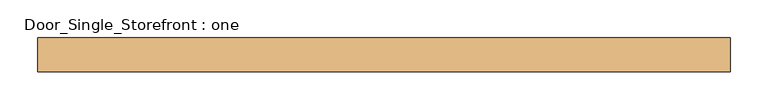
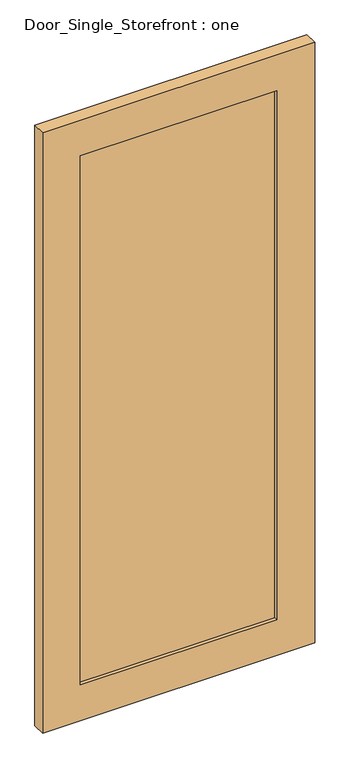
"""IFC4 building model written with IfcOpenShell, lengths in millimetres: door geometry, Door_Single_Storefront : one."""

import ifcopenshell
import ifcopenshell.guid

model = None  # the IFC model being written
_history = None  # IfcOwnerHistory: only IFC2X3 demands one
_inside = {}  # id of a spatial element -> (the spatial element, [elements in it])
_under = {}  # id of a project, library or spatial element -> (it, [spatial elements below it])
_declared = {}  # id of a project -> (the project, [libraries it declares])
_typed = {}  # id of a type object -> (the type object, [elements of that type])
_made_of = {}  # id of a material, layer set ... -> (it, [elements and type objects made of it])


def new_model(schema):
    """Start an empty IFC model of exactly this schema.

    Asked for "IFC4X3", IfcOpenShell would pick the latest addendum, in which some entities
    have other attributes; the version numbers below select the first issue.
    IFC2X3 requires an IfcOwnerHistory on every rooted entity: one is made here for all.
    """
    global model, _history
    if schema == "IFC4X3":
        model = ifcopenshell.file(schema_version=(4, 3, 0, 0))
    else:
        model = ifcopenshell.file(schema=schema)
    _inside.clear()
    _under.clear()
    _declared.clear()
    _typed.clear()
    _made_of.clear()
    _history = None
    if model.schema == "IFC2X3":
        org = make("IfcOrganization", Name="unknown")
        user = make(
            "IfcPersonAndOrganization",
            ThePerson=make("IfcPerson", FamilyName="unknown"),
            TheOrganization=org,
        )
        app = make(
            "IfcApplication",
            ApplicationDeveloper=org,
            Version="unknown",
            ApplicationFullName="unknown",
            ApplicationIdentifier="unknown",
        )
        _history = make(
            "IfcOwnerHistory",
            OwningUser=user,
            OwningApplication=app,
            ChangeAction="ADDED",
            CreationDate=0,
        )
    return model


def make(cls, **values):
    """One entity of the class cls with the attributes given. An attribute that is None is left unset."""
    return model.create_entity(
        cls, **{name: value for name, value in values.items() if value is not None}
    )


def rooted(cls, **values):
    """An entity with a GlobalId (a new one), such as an element, a storey or a relation."""
    return make(cls, GlobalId=ifcopenshell.guid.new(), OwnerHistory=_history, **values)


def si_unit(unit_type, name, prefix=None):
    """IfcSIUnit, for example si_unit("LENGTHUNIT", "METRE", prefix="MILLI")."""
    return make("IfcSIUnit", UnitType=unit_type, Prefix=prefix, Name=name)


def assignment(units):
    """IfcUnitAssignment: the units of a project."""
    return None if units is None else make("IfcUnitAssignment", Units=units)


def point(xyz):
    """IfcCartesianPoint."""
    return None if xyz is None else make("IfcCartesianPoint", Coordinates=xyz)


def direction(xyz):
    """IfcDirection."""
    return None if xyz is None else make("IfcDirection", DirectionRatios=xyz)


def frame(location, z_axis=None, x_axis=None):
    """IfcAxis2Placement3D, a coordinate frame: its origin and axes. An axis left out is left unset."""
    return make(
        "IfcAxis2Placement3D",
        Location=point(location),
        Axis=direction(z_axis),
        RefDirection=direction(x_axis),
    )


def origin():
    """The frame at (0, 0, 0) with its axes left unset."""
    return frame((0.0, 0.0, 0.0))


def place(relative_to, where):
    """IfcLocalPlacement: puts the frame where relative to a parent placement (None: the world)."""
    return make(
        "IfcLocalPlacement", PlacementRelTo=relative_to, RelativePlacement=where
    )


def context(
    kind, dimensions, precision=None, world=None, true_north=None, identifier=None
):
    """IfcGeometricRepresentationContext, for example the 3D "Model" context."""
    return make(
        "IfcGeometricRepresentationContext",
        ContextIdentifier=identifier,
        ContextType=kind,
        CoordinateSpaceDimension=dimensions,
        Precision=precision,
        WorldCoordinateSystem=world,
        TrueNorth=true_north,
    )


def project(units=None, contexts=None):
    """IfcProject with its units and contexts."""
    return rooted(
        "IfcProject",
        Name="project",
        RepresentationContexts=contexts,
        UnitsInContext=assignment(units),
    )


def spatial(cls, under=None, at=None, **own):
    """A site, building, storey or space (cls), placed at a placement, below another one or the project."""
    s = rooted(cls, ObjectPlacement=at, **own)
    if under is not None:
        _under.setdefault(under.id(), (under, []))[1].append(s)
    return s


def polyline(points):
    """IfcPolyline through the points."""
    return make("IfcPolyline", Points=[point(p) for p in points])


def outline(outer, holes=None, kind="AREA"):
    """IfcArbitraryClosedProfileDef: a profile drawn as a closed curve; with holes, ...WithVoids."""
    if holes is None:
        return make("IfcArbitraryClosedProfileDef", ProfileType=kind, OuterCurve=outer)
    return make(
        "IfcArbitraryProfileDefWithVoids",
        ProfileType=kind,
        OuterCurve=outer,
        InnerCurves=holes,
    )


def extrude(swept, where, along, depth):
    """IfcExtrudedAreaSolid: the profile swept, set in the frame where, extruded along a direction by depth."""
    return make(
        "IfcExtrudedAreaSolid",
        SweptArea=swept,
        Position=where,
        ExtrudedDirection=direction(along),
        Depth=depth,
    )


def shape(context_of_items, identifier, shape_type, items):
    """IfcShapeRepresentation: the items that make up one representation, for example the "Body"."""
    return make(
        "IfcShapeRepresentation",
        ContextOfItems=context_of_items,
        RepresentationIdentifier=identifier,
        RepresentationType=shape_type,
        Items=items,
    )


def source(mapping_origin, context_of_items, identifier, shape_type, items):
    """IfcRepresentationMap: a shape defined once, which mapped items show again and again."""
    return make(
        "IfcRepresentationMap",
        MappingOrigin=mapping_origin,
        MappedRepresentation=shape(context_of_items, identifier, shape_type, items),
    )


def transform(
    local_origin,
    x_axis=None,
    y_axis=None,
    z_axis=None,
    scale=None,
    scale2=None,
    scale3=None,
    uniform=True,
):
    """IfcCartesianTransformationOperator3D, or its non-uniform kind. x_axis, y_axis, z_axis: its Axis1, 2, 3."""
    if uniform:
        return make(
            "IfcCartesianTransformationOperator3D",
            Axis1=direction(x_axis),
            Axis2=direction(y_axis),
            LocalOrigin=point(local_origin),
            Scale=scale,
            Axis3=direction(z_axis),
        )
    return make(
        "IfcCartesianTransformationOperator3DnonUniform",
        Axis1=direction(x_axis),
        Axis2=direction(y_axis),
        LocalOrigin=point(local_origin),
        Scale=scale,
        Axis3=direction(z_axis),
        Scale2=scale2,
        Scale3=scale3,
    )


def mapped(mapping_source, mapping_target):
    """IfcMappedItem: shows the shape of a source again, moved by a transform."""
    return make(
        "IfcMappedItem", MappingSource=mapping_source, MappingTarget=mapping_target
    )


def made_of(thing, what):
    """Note that an element or type object is made of a material, layer set ...; save() writes the relation."""
    if what is not None:
        _made_of.setdefault(what.id(), (what, []))[1].append(thing)
    return thing


def element(
    cls,
    number,
    at=None,
    inside=None,
    cuts=None,
    type_object=None,
    material=None,
    context=None,
    identifier="Body",
    shape_type=None,
    held_by="IfcProductDefinitionShape",
    body=None,
    shapes=None,
    **own,
):
    """One element of the class cls, such as IfcWall. Its Tag is "e" and its number.

    at: its placement. inside: the storey or other place that contains it. cuts: it is an
    opening in that element (IfcRelVoidsElement). A single representation is given by context,
    identifier, shape_type and body (its items); several are given by shapes. held_by: the class
    of the entity that holds the representations. save() writes the other relations.
    """
    e = rooted(cls, Tag="e%d" % number, ObjectPlacement=at, **own)
    if body is not None:
        shapes = [shape(context, identifier, shape_type, body)]
    if shapes is not None:
        e.Representation = make(held_by, Representations=shapes)
    if inside is not None:
        _inside.setdefault(inside.id(), (inside, []))[1].append(e)
    if cuts is not None:
        rooted(
            "IfcRelVoidsElement", RelatingBuildingElement=cuts, RelatedOpeningElement=e
        )
    if type_object is not None:
        _typed.setdefault(type_object.id(), (type_object, []))[1].append(e)
    return made_of(e, material)


def aggregate(whole, parts):
    """IfcRelAggregates: a whole, such as a stair, and the parts it consists of."""
    return rooted("IfcRelAggregates", RelatingObject=whole, RelatedObjects=parts)


def save(model, path):
    """Write the relations noted so far, then the file.

    IfcRelAggregates (storeys below a building ...), IfcRelContainedInSpatialStructure (elements
    in a storey), IfcRelDefinesByType, IfcRelAssociatesMaterial and IfcRelDeclares: one each for
    every whole, place, type object, material and project.
    """
    for whole, parts in _under.values():
        aggregate(whole, parts)
    for where, things in _inside.values():
        rooted(
            "IfcRelContainedInSpatialStructure",
            RelatedElements=things,
            RelatingStructure=where,
        )
    for kind, things in _typed.values():
        rooted("IfcRelDefinesByType", RelatedObjects=things, RelatingType=kind)
    for what, things in _made_of.values():
        rooted("IfcRelAssociatesMaterial", RelatedObjects=things, RelatingMaterial=what)
    for by, libraries in _declared.values():
        rooted("IfcRelDeclares", RelatingContext=by, RelatedDefinitions=libraries)
    model.write(path)


def door_single_storefront_one_30533e89(model_context):
    return source(origin(), model_context, "Body", "SweptSolid", [
        extrude(outline(polyline([(330.2, -6.35), (-330.2, -6.35), (-330.2, 12.7), (330.2, 12.7), (330.2, -6.35)])), frame((0.0, 0.0, 127.0), z_axis=(0.0, 0.0, 1.0), x_axis=(1.0, 0.0, 0.0)), (0.0, 0.0, 1.0), 1879.6),
        extrude(outline(polyline([(2133.6, -457.2), (0.0, -457.2), (0.0, 457.2), (2133.6, 457.2), (2133.6, -457.2)]), holes=[polyline([(127.0, 330.2), (127.0, -330.2), (2006.6, -330.2), (2006.6, 330.2), (127.0, 330.2)])]), frame((0.0, -19.05, 0.0), z_axis=(0.0, 1.0, 0.0), x_axis=(0.0, 0.0, 1.0)), (0.0, 0.0, 1.0), 44.45),
    ])


if __name__ == "__main__":
    model = new_model("IFC4")
    model_context = context("Model", 3, world=origin())
    ifc_project = project(units=[si_unit("LENGTHUNIT", "METRE", prefix="MILLI")], contexts=[model_context])
    site = spatial("IfcSite", under=ifc_project)
    building = spatial("IfcBuilding", under=site)
    placement = place(None, origin())
    door_single_storefront_one_shape = door_single_storefront_one_30533e89(model_context)
    element("IfcDoor", 1, ObjectType="Door_Single_Storefront : one", at=placement, inside=building, context=model_context, shape_type="MappedRepresentation", body=[
        mapped(door_single_storefront_one_shape, transform((0.0, 0.0, 0.0), x_axis=(1.0, 0.0, 0.0), y_axis=(0.0, 1.0, 0.0), z_axis=(0.0, 0.0, 1.0))),
    ])
    save(model, "model.ifc")

# Revit data of these elements
# Type "Door_Single_Storefront : one"
#   Type Mark = "29"
#   Analytic Construction = "<None>"
#   Stile_Width = 0' - 5"
#   Door_Thickness = 0' - 1 3/4"
#   Door_Offset = 0' - 1"
#   Glass_Material = INSULATED GLAZING
#   Frame_Material = ALUMINUM STOREFRONT
#   Function = (empty or 0)
# Element 1 (IfcDoor, "Door_Single_Storefront : one")
#   Materials on its faces: "ALUMINUM STOREFRONT", "INSULATED GLAZING"
# Materials
#   "INSULATED GLAZING": class "Glass", colour RGB 196 205 210, transparency 0.85, Description = "Soda Lime Glass", Cost = 0
#   "ALUMINUM STOREFRONT": class "Metal", colour RGB 244 244 244, transparency 0, Description = "Aluminum 6061", Cost = 0
